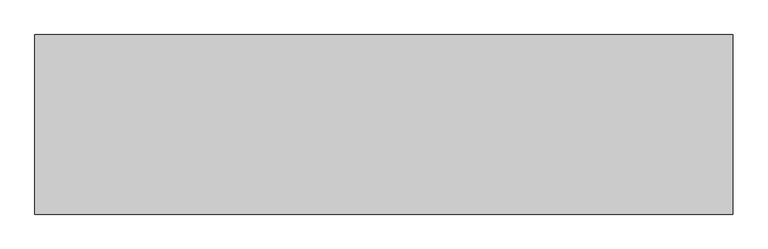
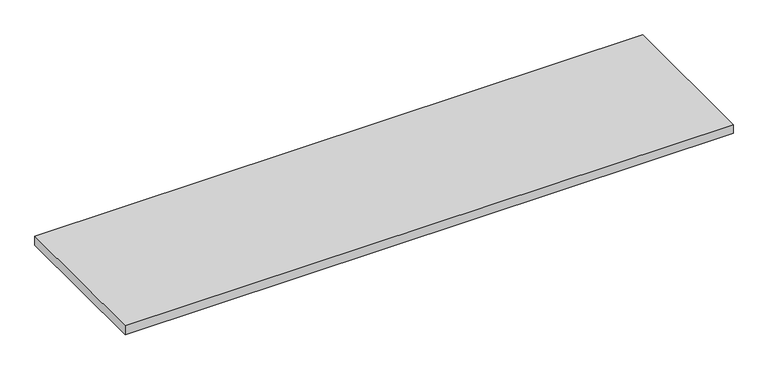
"""IFC4 building model written with IfcOpenShell, lengths in millimetres: furniture geometry, OD_CW_Countertop : OD_CW_Countertop."""

from ifc_helpers import new_model, si_unit, frame, origin, place, context, project, spatial, polyline, outline, extrude, source, transform, mapped, element, save


def furniture_f650930b(model_context):
    return source(origin(), model_context, "Body", "SweptSolid", [
        extrude(outline(polyline([(18.7377049, -609.6), (18.7377049, 25.4), (2486.9042456, 25.4), (2486.9042456, -609.6), (18.7377049, -609.6)])), frame((0.0, 0.0, 1066.8), z_axis=(0.0, 0.0, 1.0), x_axis=(1.0, 0.0, 0.0)), (0.0, 0.0, 1.0), 38.1),
    ])


if __name__ == "__main__":
    model = new_model("IFC4")
    model_context = context("Model", 3, world=origin())
    ifc_project = project(units=[si_unit("LENGTHUNIT", "METRE", prefix="MILLI")], contexts=[model_context])
    site = spatial("IfcSite", under=ifc_project)
    building = spatial("IfcBuilding", under=site)
    placement = place(None, origin())
    furniture_shape = furniture_f650930b(model_context)
    element("IfcFurniture", 1, ObjectType="OD_CW_Countertop : OD_CW_Countertop", at=placement, inside=building, context=model_context, shape_type="MappedRepresentation", body=[
        mapped(furniture_shape, transform((0.0, 0.0, 0.0), x_axis=(1.0, 0.0, 0.0), y_axis=(0.0, 1.0, 0.0), z_axis=(0.0, 0.0, 1.0))),
    ])
    save(model, "model.ifc")

# Revit data of these elements
# Type "OD_CW_Countertop : OD_CW_Countertop"
#   OD_CW_Width [instance default] = 2' - 9"
#   OD_CW_Off Floor [instance default] = 3' - 2"
#   OD_CW_Length [instance default] = 6' - 9"
#   OD_CW_Height [instance default] = 7' - 0"
#   Depth = 2' - 0"
#   Height = 3' - 0"
#   Width = 4' - 0"
#   OD_CW_Material_Countertop [instance default] = none
# Element 1 (IfcFurniture, "OD_CW_Countertop : OD_CW_Countertop")
#   OD_CW_Width = 2' - 1"
#   OD_CW_Off Floor = 3' - 6"
#   OD_CW_Length = 8' - 1.17191"
#   OD_CW_Height = 0' - 1 1/2"
#   Materials on its faces: "CASEWORK"
# Materials
#   "CASEWORK": class "Generic", colour RGB 181 181 181, transparency 0, Cost = 0
